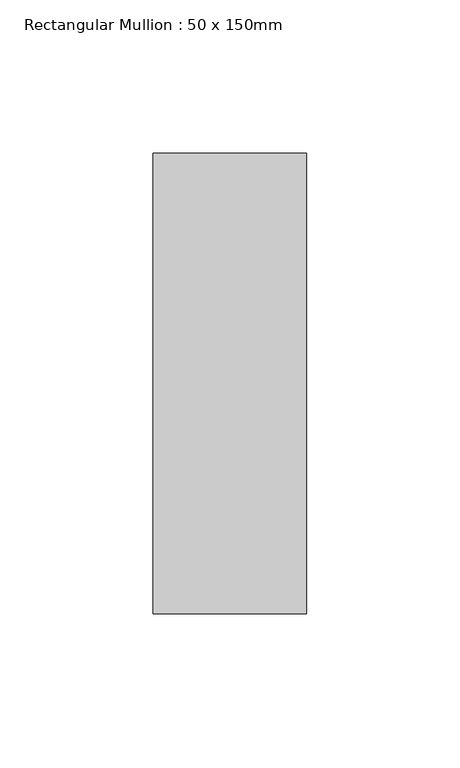
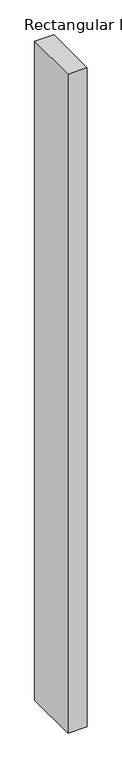
"""IFC4 building model written with IfcOpenShell, lengths in millimetres: member geometry, Rectangular Mullion : 50 x 150mm."""

from ifc_helpers import new_model, si_unit, frame, origin, place, context, project, spatial, polyline, outline, extrude, source, transform, mapped, element, save


def rectangular_mullion_50_x_150mm_c22c5d1d(model_context):
    return source(origin(), model_context, "Body", "SweptSolid", [
        extrude(outline(polyline([(25.0, 75.0), (25.0, -75.0), (-25.0, -75.0), (-25.0, 75.0), (25.0, 75.0)])), frame((0.0, 0.0, -1811.1666669), z_axis=(0.0, 0.0, 1.0), x_axis=(1.0, 0.0, 0.0)), (0.0, 0.0, 1.0), 1811.1666669),
    ])


if __name__ == "__main__":
    model = new_model("IFC4")
    model_context = context("Model", 3, world=origin())
    ifc_project = project(units=[si_unit("LENGTHUNIT", "METRE", prefix="MILLI")], contexts=[model_context])
    site = spatial("IfcSite", under=ifc_project)
    building = spatial("IfcBuilding", under=site)
    placement = place(None, origin())
    rectangular_mullion_50_x_150mm_shape = rectangular_mullion_50_x_150mm_c22c5d1d(model_context)
    element("IfcMember", 1, ObjectType="Rectangular Mullion : 50 x 150mm", at=placement, inside=building, context=model_context, shape_type="MappedRepresentation", body=[
        mapped(rectangular_mullion_50_x_150mm_shape, transform((0.0, 0.0, 0.0), x_axis=(1.0, 0.0, 0.0), y_axis=(0.0, 1.0, 0.0), z_axis=(0.0, 0.0, 1.0))),
    ])
    save(model, "model.ifc")

# Revit data of these elements
# Type "Rectangular Mullion : 50 x 150mm"
#   built-in parameter 1007304 = 0.492126 (stored number, unit not read)
#   built-in parameter 1007301 = 0.082021 (stored number, unit not read)
#   built-in parameter 1007300 = 0.082021 (stored number, unit not read)
# Element 1 (IfcMember, "Rectangular Mullion : 50 x 150mm")
#   Materials on its faces: "Metal - Aluminium"
# Materials
#   "Metal - Aluminium": class "Metal", colour RGB 247 247 247, transparency 0
